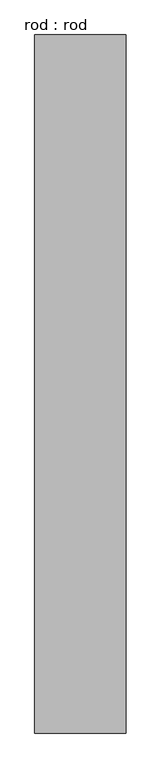
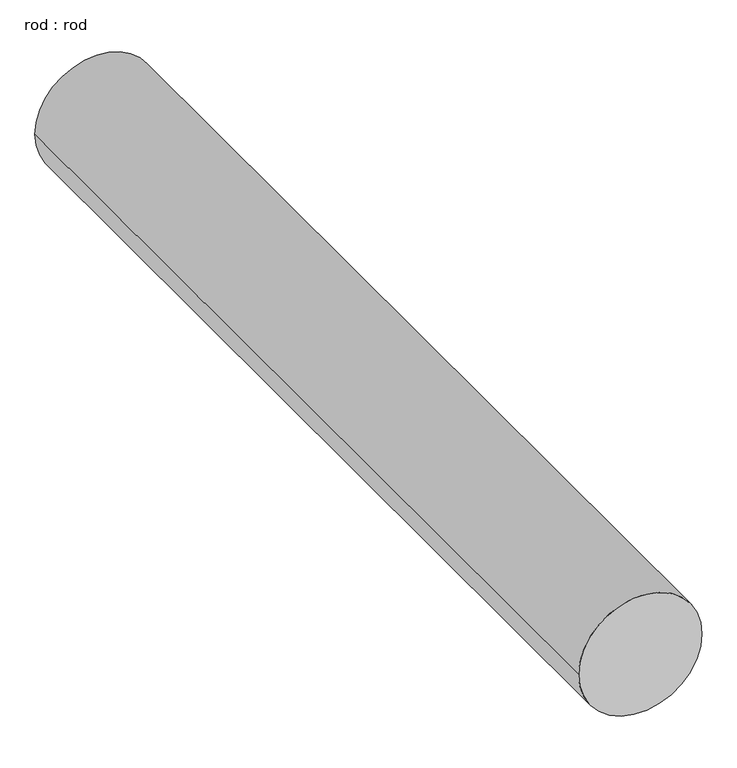
"""IFC4 building model written with IfcOpenShell, lengths in millimetres: proxy geometry, rod : rod."""

from ifc_helpers import new_model, si_unit, point, frame, frame_2d, origin, place, context, project, spatial, circle_curve, trimmed, segment, composite_curve, outline, extrude, source, transform, mapped, element, save


def rod_rod_7b2b5b40(model_context):
    return source(origin(), model_context, "Body", "SweptSolid", [
        extrude(outline(composite_curve([segment(trimmed(circle_curve(frame_2d((0.0108462, 0.0)), 200.0), [point((0.0108462, 200.0))], [point((0.0108462, -200.0))], False, "CARTESIAN"), True, "CONTINUOUS"), segment(trimmed(circle_curve(frame_2d((0.0108462, 0.0)), 200.0), [point((0.0108462, -200.0))], [point((0.0108462, 200.0))], False, "CARTESIAN"), True, "CONTINUOUS")], self_intersect=False)), frame((0.0, 2565.9429011, 0.0), z_axis=(0.0, 1.0, 0.0), x_axis=(0.0, 0.0, 1.0)), (0.0, 0.0, 1.0), 3053.5714286),
    ])


if __name__ == "__main__":
    model = new_model("IFC4")
    model_context = context("Model", 3, world=origin())
    ifc_project = project(units=[si_unit("LENGTHUNIT", "METRE", prefix="MILLI")], contexts=[model_context])
    site = spatial("IfcSite", under=ifc_project)
    building = spatial("IfcBuilding", under=site)
    placement = place(None, origin())
    rod_rod_shape = rod_rod_7b2b5b40(model_context)
    element("IfcBuildingElementProxy", 1, Name="rod : rod", ObjectType="rod : rod", at=placement, inside=building, context=model_context, shape_type="MappedRepresentation", body=[
        mapped(rod_rod_shape, transform((0.0, 0.0, 0.0), x_axis=(1.0, 0.0, 0.0), y_axis=(0.0, 1.0, 0.0), z_axis=(0.0, 0.0, 1.0))),
    ])
    save(model, "model.ifc")

# Revit data of these elements
# Type "rod : rod"
#   Default Elevation = 0
